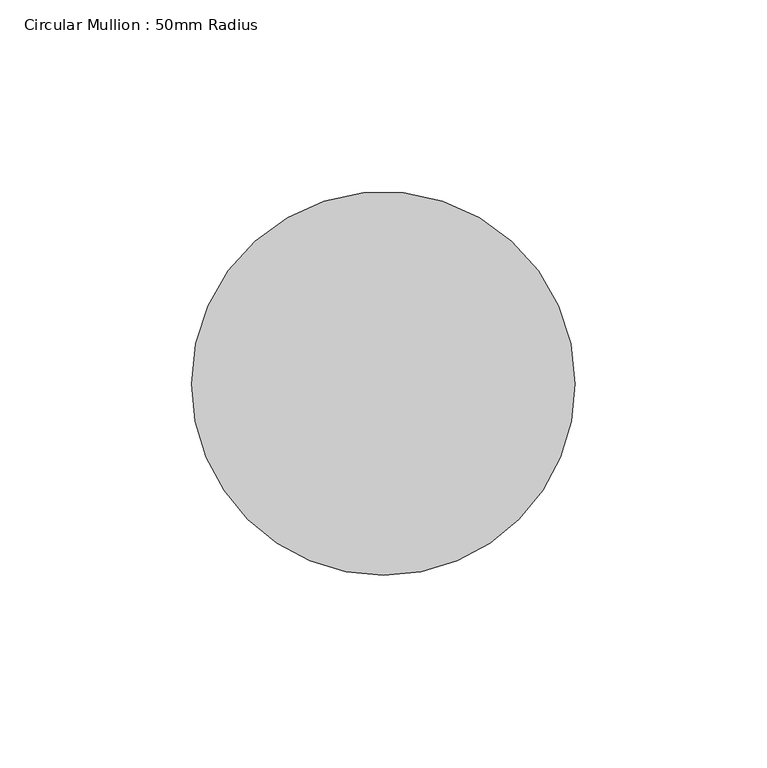
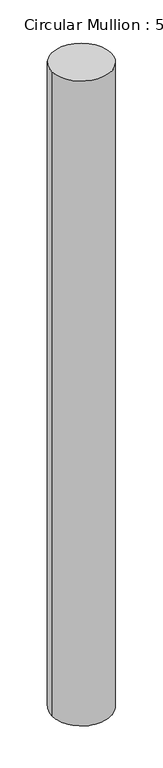
"""IFC4 building model written with IfcOpenShell, lengths in millimetres: member geometry, Circular Mullion : 50mm Radius."""

from ifc_helpers import new_model, si_unit, frame, origin, place, context, project, spatial, ellipse_curve, source, transform, mapped, element, save
from ifc_brep_helpers import plane_surface, cylinder_surface, advanced_brep


def circular_mullion_50mm_radius_230a32d0(model_context):
    return source(origin(), model_context, "Body", "AdvancedBrep", [
        advanced_brep(
        [(-100.0, 0.0, 1.0709921), (0.0, 0.0, 0.0), (0.0, 0.0, -1151.826771), (-100.0, 0.0, -1152.9602073)],
        [
            (0, 1, ellipse_curve(frame((-50.0, 0.0, 0.5354961), z_axis=(-0.010707170245775843, -0.019975787037388733, -0.9997431292274856), x_axis=(-0.4723008026464624, -0.8811460016688908, 0.022664411804298436)), 50.0128468, 50.0)),
            (1, 2),
            (2, 3, ellipse_curve(frame((-50.0, 0.0, -1152.3934891), z_axis=(-0.011331102082938646, -0.02113982283946596, 0.9997123156268019), x_axis=(0.47228624561883875, 0.8811188434116958, 0.02398512005593206)), 50.0143884, 50.0)),
            (3, 0),
            (1, 0, ellipse_curve(frame((-50.0, 0.0, 0.5354961), z_axis=(-0.010707170245775843, -0.019975787037388733, -0.9997431292274856), x_axis=(-0.4723008026464624, -0.8811460016688908, 0.022664411804298436)), 50.0128468, 50.0)),
            (3, 2, ellipse_curve(frame((-50.0, 0.0, -1152.3934891), z_axis=(-0.011331102082938646, -0.02113982283946596, 0.9997123156268019), x_axis=(0.47228624561883875, 0.8811188434116958, 0.02398512005593206)), 50.0143884, 50.0)),
        ],
        [
            cylinder_surface(frame((-50.0, 0.0, 0.0), z_axis=(0.0, 0.0, 1.0), x_axis=(1.0, 0.0, 0.0)), 50.0),
            plane_surface(frame((-268.6423077, 143.9942726, 0.0), z_axis=(0.010707170245775843, 0.019975787037388733, 0.9997431292274856), x_axis=(0.47230080264646435, 0.8811460016688895, -0.02266441180430534))),
            plane_surface(frame((-268.6423077, 143.9942726, -1151.826771), z_axis=(0.011331102082938646, 0.02113982283946596, -0.9997123156268019), x_axis=(0.4722862456188387, 0.8811188434116956, 0.023985120055942666))),
        ],
        [
            (0, [[1, 2, 3, 4]]),
            (0, [[5, -4, 6, -2]]),
            (1, [[-1, -5]]),
            (2, [[-6, -3]]),
        ],
    ),
    ])


if __name__ == "__main__":
    model = new_model("IFC4")
    model_context = context("Model", 3, world=origin())
    ifc_project = project(units=[si_unit("LENGTHUNIT", "METRE", prefix="MILLI")], contexts=[model_context])
    site = spatial("IfcSite", under=ifc_project)
    building = spatial("IfcBuilding", under=site)
    placement = place(None, origin())
    circular_mullion_50mm_radius_shape = circular_mullion_50mm_radius_230a32d0(model_context)
    element("IfcMember", 1, ObjectType="Circular Mullion : 50mm Radius", at=placement, inside=building, context=model_context, shape_type="MappedRepresentation", body=[
        mapped(circular_mullion_50mm_radius_shape, transform((0.0, 0.0, 0.0), x_axis=(1.0, 0.0, 0.0), y_axis=(0.0, 1.0, 0.0), z_axis=(0.0, 0.0, 1.0))),
    ])
    save(model, "model.ifc")

# Revit data of these elements
# Type "Circular Mullion : 50mm Radius"
#   built-in parameter 1007350 = 0.164042 (stored number, unit not read)
# Element 1 (IfcMember, "Circular Mullion : 50mm Radius")
#   Materials on its faces: "Aluminium"
# Materials
#   "Aluminium": class "Metal", colour RGB 247 247 247, transparency 0, Description = "Aluminium 6061", Cost = 0
